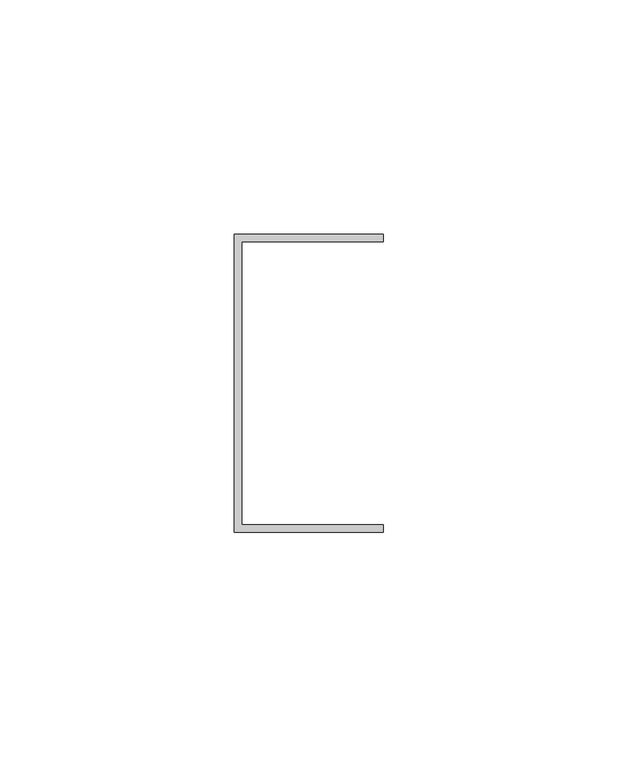
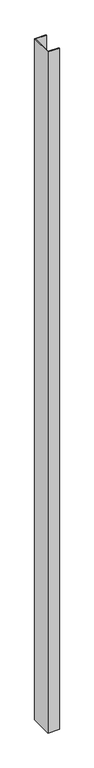
"""IFC4 building model written with IfcOpenShell, lengths in millimetres: proxy geometry, Generic Models 7:Generic Models 1:3:Generic Models 1:3 : Generic Models 7:Generic Models 1:305549:3:Generic Models 1:3:Generic Models 1:3 : Generic Models 7:Generic Models 1:305549:3 : Generic Models 7:Generic Models 1:3:Generic Models 1:3 : Generic Models 7:Generic Models 1:305549:301244:46 : Generic Models 7:Generic Models 1:3:Generic Models 1:3 : Generic Models 7:Generic Models 1:305549:3:Generic Models 1:3:Generic Models 1:3 : Generic Models 7:Generic Models 1:305549:3 : Generic Models 7:Generic Models 1:3:Generic Models 1:3 : Generic Models 7:Generic Models 1:305549:301244:308848."""

from ifc_helpers import new_model, si_unit, frame, origin, place, context, project, spatial, polyline, outline, extrude, source, transform, mapped, element, save


def generic_models_43a98676(model_context):
    return source(origin(), model_context, "Body", "SweptSolid", [
        extrude(outline(polyline([(803177.9632437, -579013.3913841), (803209.7132437, -579013.3913841), (803209.7132437, -579014.9788841), (803179.5507437, -579014.9788841), (803179.5507437, -579075.3038841), (803209.7132437, -579075.3038841), (803209.7132437, -579076.8913841), (803177.9632437, -579076.8913841), (803177.9632437, -579013.3913841)])), frame((0.0, 0.0, 4133.81326), z_axis=(0.0, 0.0, 1.0), x_axis=(1.0, 0.0, 0.0)), (0.0, 0.0, 1.0), 2000.28674),
    ])


if __name__ == "__main__":
    model = new_model("IFC4")
    model_context = context("Model", 3, world=origin())
    ifc_project = project(units=[si_unit("LENGTHUNIT", "METRE", prefix="MILLI")], contexts=[model_context])
    site = spatial("IfcSite", under=ifc_project)
    building = spatial("IfcBuilding", under=site)
    placement = place(None, origin())
    generic_models_shape = generic_models_43a98676(model_context)
    element("IfcBuildingElementProxy", 1, Name="Generic Models 7:Generic Models 1:3:Generic Models 1:3 : Generic Models 7:Generic Models 1:305549:3:Generic Models 1:3:Generic Models 1:3 : Generic Models 7:Generic Models 1:305549:3 : Generic Models 7:Generic Models 1:3:Generic Models 1:3 : Generic Models 7:Generic Models 1:305549:301244:46 : Generic Models 7:Generic Models 1:3:Generic Models 1:3 : Generic Models 7:Generic Models 1:305549:3:Generic Models 1:3:Generic Models 1:3 : Generic Models 7:Generic Models 1:305549:3 : Generic Models 7:Generic Models 1:3:Generic Models 1:3 : Generic Models 7:Generic Models 1:305549:301244:308848", ObjectType="Generic Models 7:Generic Models 1:3:Generic Models 1:3 : Generic Models 7:Generic Models 1:305549:3:Generic Models 1:3:Generic Models 1:3 : Generic Models 7:Generic Models 1:305549:3 : Generic Models 7:Generic Models 1:3:Generic Models 1:3 : Generic Models 7:Generic Models 1:305549:301244:46 : Generic Models 7:Generic Models 1:3:Generic Models 1:3 : Generic Models 7:Generic Models 1:305549:3:Generic Models 1:3:Generic Models 1:3 : Generic Models 7:Generic Models 1:305549:3 : Generic Models 7:Generic Models 1:3:Generic Models 1:3 : Generic Models 7:Generic Models 1:305549:301244:308848", at=placement, inside=building, context=model_context, shape_type="MappedRepresentation", body=[
        mapped(generic_models_shape, transform((0.0, 0.0, 0.0), x_axis=(1.0, 0.0, 0.0), y_axis=(0.0, 1.0, 0.0), z_axis=(0.0, 0.0, 1.0))),
    ])
    save(model, "model.ifc")

# Revit data of these elements
# Type "Generic Models 7:Generic Models 1:3:Generic Models 1:3 : Generic Models 7:Generic Models 1:305549:3:Generic Models 1:3:Generic Models 1:3 : Generic Models 7:Generic Models 1:305549:3 : Generic Models 7:Generic Models 1:3:Generic Models 1:3 : Generic Models 7:Generic Models 1:305549:301244:46 : Generic Models 7:Generic Models 1:3:Generic Models 1:3 : Generic Models 7:Generic Models 1:305549:3:Generic Models 1:3:Generic Models 1:3 : Generic Models 7:Generic Models 1:305549:3 : Generic Models 7:Generic Models 1:3:Generic Models 1:3 : Generic Models 7:Generic Models 1:305549:301244:308848"
#   NameOverride = "Generic Models 7:Generic Models 1:3:Generic Models 1:3 : Generic Models 7:Generic Models 1:305549:3:Generic Models 1:3:Generic Models 1:3 : Generic Models 7:Generic Models 1:305549:3 : Generic Models 7:Generic Models 1:3:Generic Models 1:3 : Generic Models 7:Generic Models 1:305549:301244:308848"
#   ObjectTypeOverride = "Generic Models 1:3:Generic Models 1:3 : Generic Models 7:Generic Models 1:305549:3 : Generic Models 7:Generic Models 1:3:Generic Models 1:3 : Generic Models 7:Generic Models 1:305549:301244"
#   Reference = "Generic Models 1"
#   Tag = "308848"
# Element 1 (IfcBuildingElementProxy, "Generic Models 7:Generic Models 1:3:Generic Models 1:3 : Generic Models 7:Generic Models 1:305549:3:Generic Models 1:3:Generic Models 1:3 : Generic Models 7:Generic Models 1:305549:3 : Generic Models 7:Generic Models 1:3:Generic Models 1:3 : Generic Models 7:Generic Models 1:305549:301244:46 : Generic Models 7:Generic Models 1:3:Generic Models 1:3 : Generic Models 7:Generic Models 1:305549:3:Generic Models 1:3:Generic Models 1:3 : Generic Models 7:Generic Models 1:305549:3 : Generic Models 7:Generic Models 1:3:Generic Models 1:3 : Generic Models 7:Generic Models 1:305549:301244:308848")
#   Materials on its faces: "GALVANIZED U-CHANNEL (250T125-33)"
# Materials
#   "GALVANIZED U-CHANNEL (250T125-33)": class "Unassigned", colour RGB 202 201 200, transparency 0, Keynote = "M05451300.02", Cost = 0
